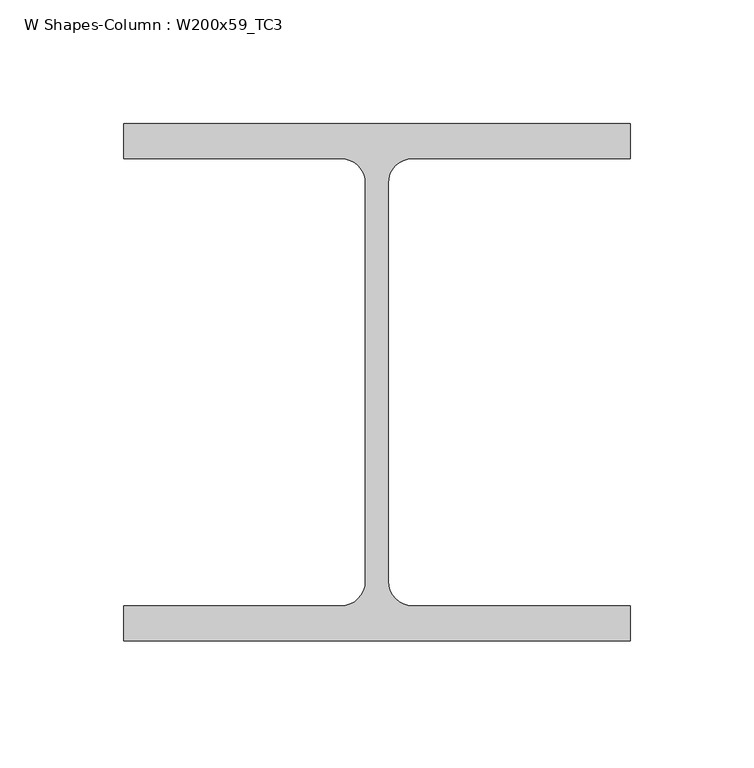
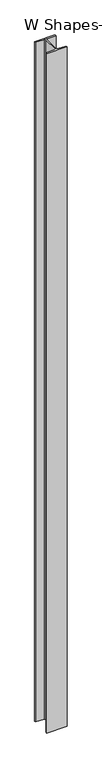
"""IFC4 building model written with IfcOpenShell, lengths in millimetres: column geometry, W Shapes-Column : W200x59_TC3."""

from ifc_helpers import new_model, si_unit, point, frame, frame_2d, origin, place, context, project, spatial, polyline, circle_curve, trimmed, segment, composite_curve, outline, extrude, source, transform, mapped, element, save


def w_shapes_column_w200x59_tc3_db71346a(model_context):
    return source(origin(), model_context, "Body", "SweptSolid", [
        extrude(outline(composite_curve([segment(polyline([(102.489, -104.775), (-102.489, -104.775), (-102.489, -90.551), (-14.5796, -90.551)]), True, "CONTINUOUS"), segment(trimmed(circle_curve(frame_2d((-14.5796, -80.5434)), 10.0076), [point((-14.5796, -90.551))], [point((-4.572, -80.5434))], True, "CARTESIAN"), True, "CONTINUOUS"), segment(polyline([(-4.572, -80.5434), (-4.572, 80.5434)]), True, "CONTINUOUS"), segment(trimmed(circle_curve(frame_2d((-14.5796, 80.5434)), 10.0076), [point((-4.572, 80.5434))], [point((-14.5796, 90.551))], True, "CARTESIAN"), True, "CONTINUOUS"), segment(polyline([(-14.5796, 90.551), (-102.489, 90.551), (-102.489, 104.775), (102.489, 104.775), (102.489, 90.551), (14.5796, 90.551)]), True, "CONTINUOUS"), segment(trimmed(circle_curve(frame_2d((14.5796, 80.5434)), 10.0076), [point((14.5796, 90.551))], [point((4.572, 80.5434))], True, "CARTESIAN"), True, "CONTINUOUS"), segment(polyline([(4.572, 80.5434), (4.572, -80.5434)]), True, "CONTINUOUS"), segment(trimmed(circle_curve(frame_2d((14.5796, -80.5434)), 10.0076), [point((4.572, -80.5434))], [point((14.5796, -90.551))], True, "CARTESIAN"), True, "CONTINUOUS"), segment(polyline([(14.5796, -90.551), (102.489, -90.551), (102.489, -104.775)]), True, "CONTINUOUS")], self_intersect=False)), frame((0.0, 0.0, 200.0), z_axis=(0.0, 0.0, 1.0), x_axis=(1.0, 0.0, 0.0)), (0.0, 0.0, 1.0), 7250.0),
    ])


if __name__ == "__main__":
    model = new_model("IFC4")
    model_context = context("Model", 3, world=origin())
    ifc_project = project(units=[si_unit("LENGTHUNIT", "METRE", prefix="MILLI")], contexts=[model_context])
    site = spatial("IfcSite", under=ifc_project)
    building = spatial("IfcBuilding", under=site)
    placement = place(None, origin())
    w_shapes_column_w200x59_tc3_shape = w_shapes_column_w200x59_tc3_db71346a(model_context)
    element("IfcColumn", 1, ObjectType="W Shapes-Column : W200x59_TC3", at=placement, inside=building, context=model_context, shape_type="MappedRepresentation", body=[
        mapped(w_shapes_column_w200x59_tc3_shape, transform((0.0, 0.0, 0.0), x_axis=(1.0, 0.0, 0.0), y_axis=(0.0, 1.0, 0.0), z_axis=(0.0, 0.0, 1.0))),
    ])
    save(model, "model.ifc")

# Revit data of these elements
# Type "W Shapes-Column : W200x59_TC3"
#   Section Name Key = "W8X40"
#   Assembly Code = "B10"
#   Width = 20.4978 cm
#   Web Thickness = 0.9144 cm
#   Web Fillet = 1.0008 cm
#   Warping Constant = 194957.0 cm⁶
#   Torsional Moment of Inertia = 46.6179 cm⁴
#   Section Area = 75.4837 cm²
#   Plastic Modulus weak axis = 303.161 cm³
#   Plastic Modulus strong axis = 652.205 cm³
#   Perimeter = 1.20396 m²/m
#   Nominal Weight = 59.5266 kgf/m
#   Moment of Inertia weak axis = 2043.70 cm⁴
#   Moment of Inertia strong axis = 6076.98 cm⁴
#   Height = 20.955 cm
#   Flange Thickness = 1.4224 cm
#   Elastic Modulus weak axis = 199.922 cm³
#   Elastic Modulus strong axis = 581.741 cm³
#   Clear Web Height = 14.605 cm
#   Centroid Vertical = 10.4775 cm
#   Centroid Horizontal = 10.2489 cm
#   Bolt Spacing = 13.97 cm
#   Structural Material [instance default] = Steel ASTM A992
#   Principal Axes Angle = 0
# Element 1 (IfcColumn, "W Shapes-Column : W200x59_TC3")
#   Structural Material = none
# Materials
#   "Steel ASTM A992": class "Metal", colour RGB 199 199 199, transparency 0, Description = "Structural steel 50ksi", Cost = 0
